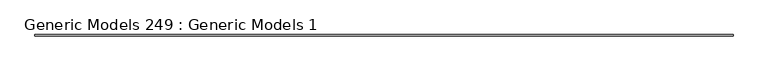
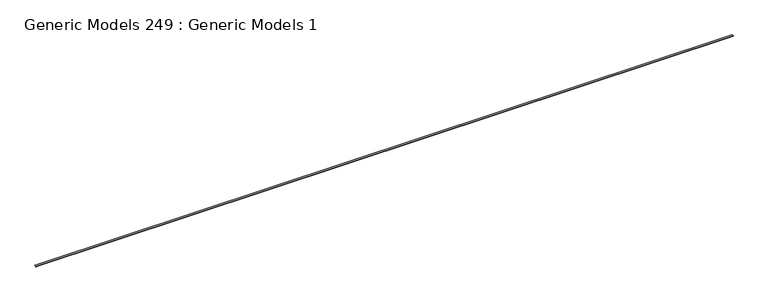
"""IFC4 building model written with IfcOpenShell, lengths in millimetres: proxy geometry, Generic Models 249 : Generic Models 1."""

import ifcopenshell
import ifcopenshell.guid

model = None  # the IFC model being written
_history = None  # IfcOwnerHistory: only IFC2X3 demands one
_inside = {}  # id of a spatial element -> (the spatial element, [elements in it])
_under = {}  # id of a project, library or spatial element -> (it, [spatial elements below it])
_declared = {}  # id of a project -> (the project, [libraries it declares])
_typed = {}  # id of a type object -> (the type object, [elements of that type])
_made_of = {}  # id of a material, layer set ... -> (it, [elements and type objects made of it])


def new_model(schema):
    """Start an empty IFC model of exactly this schema.

    Asked for "IFC4X3", IfcOpenShell would pick the latest addendum, in which some entities
    have other attributes; the version numbers below select the first issue.
    IFC2X3 requires an IfcOwnerHistory on every rooted entity: one is made here for all.
    """
    global model, _history
    if schema == "IFC4X3":
        model = ifcopenshell.file(schema_version=(4, 3, 0, 0))
    else:
        model = ifcopenshell.file(schema=schema)
    _inside.clear()
    _under.clear()
    _declared.clear()
    _typed.clear()
    _made_of.clear()
    _history = None
    if model.schema == "IFC2X3":
        org = make("IfcOrganization", Name="unknown")
        user = make(
            "IfcPersonAndOrganization",
            ThePerson=make("IfcPerson", FamilyName="unknown"),
            TheOrganization=org,
        )
        app = make(
            "IfcApplication",
            ApplicationDeveloper=org,
            Version="unknown",
            ApplicationFullName="unknown",
            ApplicationIdentifier="unknown",
        )
        _history = make(
            "IfcOwnerHistory",
            OwningUser=user,
            OwningApplication=app,
            ChangeAction="ADDED",
            CreationDate=0,
        )
    return model


def make(cls, **values):
    """One entity of the class cls with the attributes given. An attribute that is None is left unset."""
    return model.create_entity(
        cls, **{name: value for name, value in values.items() if value is not None}
    )


def rooted(cls, **values):
    """An entity with a GlobalId (a new one), such as an element, a storey or a relation."""
    return make(cls, GlobalId=ifcopenshell.guid.new(), OwnerHistory=_history, **values)


def si_unit(unit_type, name, prefix=None):
    """IfcSIUnit, for example si_unit("LENGTHUNIT", "METRE", prefix="MILLI")."""
    return make("IfcSIUnit", UnitType=unit_type, Prefix=prefix, Name=name)


def assignment(units):
    """IfcUnitAssignment: the units of a project."""
    return None if units is None else make("IfcUnitAssignment", Units=units)


def point(xyz):
    """IfcCartesianPoint."""
    return None if xyz is None else make("IfcCartesianPoint", Coordinates=xyz)


def direction(xyz):
    """IfcDirection."""
    return None if xyz is None else make("IfcDirection", DirectionRatios=xyz)


def frame(location, z_axis=None, x_axis=None):
    """IfcAxis2Placement3D, a coordinate frame: its origin and axes. An axis left out is left unset."""
    return make(
        "IfcAxis2Placement3D",
        Location=point(location),
        Axis=direction(z_axis),
        RefDirection=direction(x_axis),
    )


def origin():
    """The frame at (0, 0, 0) with its axes left unset."""
    return frame((0.0, 0.0, 0.0))


def place(relative_to, where):
    """IfcLocalPlacement: puts the frame where relative to a parent placement (None: the world)."""
    return make(
        "IfcLocalPlacement", PlacementRelTo=relative_to, RelativePlacement=where
    )


def context(
    kind, dimensions, precision=None, world=None, true_north=None, identifier=None
):
    """IfcGeometricRepresentationContext, for example the 3D "Model" context."""
    return make(
        "IfcGeometricRepresentationContext",
        ContextIdentifier=identifier,
        ContextType=kind,
        CoordinateSpaceDimension=dimensions,
        Precision=precision,
        WorldCoordinateSystem=world,
        TrueNorth=true_north,
    )


def project(units=None, contexts=None):
    """IfcProject with its units and contexts."""
    return rooted(
        "IfcProject",
        Name="project",
        RepresentationContexts=contexts,
        UnitsInContext=assignment(units),
    )


def spatial(cls, under=None, at=None, **own):
    """A site, building, storey or space (cls), placed at a placement, below another one or the project."""
    s = rooted(cls, ObjectPlacement=at, **own)
    if under is not None:
        _under.setdefault(under.id(), (under, []))[1].append(s)
    return s


def faces_of(points, faces, orient=None, outer=None):
    """IfcFace entities. A face is a list of loops; a loop is a list of indices into points, from 0.

    orient and outer hold one flag for each loop. By default every Orientation is true, the
    first loop of a face is its IfcFaceOuterBound and the others are IfcFaceBound.
    """
    made = []
    for i, loops in enumerate(faces):
        bounds = []
        for j, loop in enumerate(loops):
            is_outer = j == 0 if outer is None else outer[i][j]
            bounds.append(
                make(
                    "IfcFaceOuterBound" if is_outer else "IfcFaceBound",
                    Bound=make("IfcPolyLoop", Polygon=[points[k] for k in loop]),
                    Orientation=True if orient is None else orient[i][j],
                )
            )
        made.append(make("IfcFace", Bounds=bounds))
    return made


def faceted_brep(points, faces, orient=None, outer=None, voids=None):
    """IfcFacetedBrep: a solid bounded by flat faces; with voids (closed shells), ...WithVoids."""
    shared = [point(p) for p in points]
    hull = make("IfcClosedShell", CfsFaces=faces_of(shared, faces, orient, outer))
    if voids is None:
        return make("IfcFacetedBrep", Outer=hull)
    return make(
        "IfcFacetedBrepWithVoids",
        Outer=hull,
        Voids=[
            make(cls, CfsFaces=faces_of(shared, fs, o, b)) for cls, fs, o, b in voids
        ],
    )


def shape(context_of_items, identifier, shape_type, items):
    """IfcShapeRepresentation: the items that make up one representation, for example the "Body"."""
    return make(
        "IfcShapeRepresentation",
        ContextOfItems=context_of_items,
        RepresentationIdentifier=identifier,
        RepresentationType=shape_type,
        Items=items,
    )


def source(mapping_origin, context_of_items, identifier, shape_type, items):
    """IfcRepresentationMap: a shape defined once, which mapped items show again and again."""
    return make(
        "IfcRepresentationMap",
        MappingOrigin=mapping_origin,
        MappedRepresentation=shape(context_of_items, identifier, shape_type, items),
    )


def transform(
    local_origin,
    x_axis=None,
    y_axis=None,
    z_axis=None,
    scale=None,
    scale2=None,
    scale3=None,
    uniform=True,
):
    """IfcCartesianTransformationOperator3D, or its non-uniform kind. x_axis, y_axis, z_axis: its Axis1, 2, 3."""
    if uniform:
        return make(
            "IfcCartesianTransformationOperator3D",
            Axis1=direction(x_axis),
            Axis2=direction(y_axis),
            LocalOrigin=point(local_origin),
            Scale=scale,
            Axis3=direction(z_axis),
        )
    return make(
        "IfcCartesianTransformationOperator3DnonUniform",
        Axis1=direction(x_axis),
        Axis2=direction(y_axis),
        LocalOrigin=point(local_origin),
        Scale=scale,
        Axis3=direction(z_axis),
        Scale2=scale2,
        Scale3=scale3,
    )


def mapped(mapping_source, mapping_target):
    """IfcMappedItem: shows the shape of a source again, moved by a transform."""
    return make(
        "IfcMappedItem", MappingSource=mapping_source, MappingTarget=mapping_target
    )


def made_of(thing, what):
    """Note that an element or type object is made of a material, layer set ...; save() writes the relation."""
    if what is not None:
        _made_of.setdefault(what.id(), (what, []))[1].append(thing)
    return thing


def element(
    cls,
    number,
    at=None,
    inside=None,
    cuts=None,
    type_object=None,
    material=None,
    context=None,
    identifier="Body",
    shape_type=None,
    held_by="IfcProductDefinitionShape",
    body=None,
    shapes=None,
    **own,
):
    """One element of the class cls, such as IfcWall. Its Tag is "e" and its number.

    at: its placement. inside: the storey or other place that contains it. cuts: it is an
    opening in that element (IfcRelVoidsElement). A single representation is given by context,
    identifier, shape_type and body (its items); several are given by shapes. held_by: the class
    of the entity that holds the representations. save() writes the other relations.
    """
    e = rooted(cls, Tag="e%d" % number, ObjectPlacement=at, **own)
    if body is not None:
        shapes = [shape(context, identifier, shape_type, body)]
    if shapes is not None:
        e.Representation = make(held_by, Representations=shapes)
    if inside is not None:
        _inside.setdefault(inside.id(), (inside, []))[1].append(e)
    if cuts is not None:
        rooted(
            "IfcRelVoidsElement", RelatingBuildingElement=cuts, RelatedOpeningElement=e
        )
    if type_object is not None:
        _typed.setdefault(type_object.id(), (type_object, []))[1].append(e)
    return made_of(e, material)


def aggregate(whole, parts):
    """IfcRelAggregates: a whole, such as a stair, and the parts it consists of."""
    return rooted("IfcRelAggregates", RelatingObject=whole, RelatedObjects=parts)


def save(model, path):
    """Write the relations noted so far, then the file.

    IfcRelAggregates (storeys below a building ...), IfcRelContainedInSpatialStructure (elements
    in a storey), IfcRelDefinesByType, IfcRelAssociatesMaterial and IfcRelDeclares: one each for
    every whole, place, type object, material and project.
    """
    for whole, parts in _under.values():
        aggregate(whole, parts)
    for where, things in _inside.values():
        rooted(
            "IfcRelContainedInSpatialStructure",
            RelatedElements=things,
            RelatingStructure=where,
        )
    for kind, things in _typed.values():
        rooted("IfcRelDefinesByType", RelatedObjects=things, RelatingType=kind)
    for what, things in _made_of.values():
        rooted("IfcRelAssociatesMaterial", RelatedObjects=things, RelatingMaterial=what)
    for by, libraries in _declared.values():
        rooted("IfcRelDeclares", RelatingContext=by, RelatedDefinitions=libraries)
    model.write(path)


def generic_models_249_generic_models_1_f155bf51(model_context):
    return source(origin(), model_context, "Body", "Brep", [
        faceted_brep([(-5248.1628079, -20261.4171024, 126780.671), (-5248.1628079, -20261.4171024, 126802.896), (-5248.1628079, -20223.3171024, 126802.896), (-5248.1628079, -20223.3171024, 126801.626), (-5248.1628079, -20260.1471024, 126801.626), (-5248.1628079, -20260.1471024, 126781.941), (-5248.1628079, -20257.9373024, 126781.941), (-5248.1628079, -20257.9373024, 126783.6734564), (-5248.1628079, -20256.6673024, 126783.6734564), (-5248.1628079, -20256.6673024, 126780.671), (13801.8371921, -20261.4171024, 126780.671), (13801.8371921, -20256.6673024, 126780.671), (13801.8371921, -20256.6673024, 126783.6734564), (13801.8371921, -20257.9373024, 126783.6734564), (13801.8371921, -20257.9373024, 126781.941), (13801.8371921, -20260.1471024, 126781.941), (13801.8371921, -20260.1471024, 126801.626), (13801.8371921, -20223.3171024, 126801.626), (13801.8371921, -20223.3171024, 126802.896), (13801.8371921, -20261.4171024, 126802.896), (13593.8187142, -20223.3171024, 126802.896), (-5049.7812858, -20223.3171024, 126802.896), (13593.8187142, -20223.3171024, 126801.626), (-5049.7812858, -20223.3171024, 126801.626), (13593.8187142, -20260.1471024, 126801.626), (-5049.7812858, -20260.1471024, 126801.626), (13593.8187142, -20260.1471024, 126781.941), (-5049.7812858, -20260.1471024, 126781.941), (13593.8187142, -20257.9373024, 126781.941), (-5049.7812858, -20257.9373024, 126781.941), (-5049.7812858, -20257.9373024, 126783.6734564), (13593.8187142, -20257.9373024, 126783.6734564), (13593.8187142, -20256.6673024, 126783.6734564), (-5049.7812858, -20256.6673024, 126783.6734564), (13593.8187142, -20256.6673024, 126780.671), (-5049.7812858, -20256.6673024, 126780.671)], [[[0, 1, 2, 3, 4, 5, 6, 7, 8, 9]], [[10, 11, 12, 13, 14, 15, 16, 17, 18, 19]], [[1, 0, 10, 19]], [[2, 1, 19, 18, 20, 21]], [[3, 2, 21, 20, 18, 17, 22, 23]], [[4, 3, 23, 22, 17, 16, 24, 25]], [[5, 4, 25, 24, 16, 15, 26, 27]], [[6, 5, 27, 26, 15, 14, 28, 29]], [[8, 7, 30, 31, 13, 12, 32, 33]], [[9, 8, 33, 32, 12, 11, 34, 35]], [[0, 9, 35, 34, 11, 10]], [[7, 6, 29, 28, 14, 13, 31, 30]]]),
    ])


if __name__ == "__main__":
    model = new_model("IFC4")
    model_context = context("Model", 3, world=origin())
    ifc_project = project(units=[si_unit("LENGTHUNIT", "METRE", prefix="MILLI")], contexts=[model_context])
    site = spatial("IfcSite", under=ifc_project)
    building = spatial("IfcBuilding", under=site)
    placement = place(None, origin())
    generic_models_249_generic_models_1_shape = generic_models_249_generic_models_1_f155bf51(model_context)
    element("IfcBuildingElementProxy", 1, Name="Generic Models 249 : Generic Models 1", ObjectType="Generic Models 249 : Generic Models 1", at=placement, inside=building, context=model_context, shape_type="MappedRepresentation", body=[
        mapped(generic_models_249_generic_models_1_shape, transform((0.0, 0.0, 0.0), x_axis=(1.0, 0.0, 0.0), y_axis=(0.0, 1.0, 0.0), z_axis=(0.0, 0.0, 1.0))),
    ])
    save(model, "model.ifc")

# Revit data of these elements
# Element 1 (IfcBuildingElementProxy, "Generic Models 249 : Generic Models 1")
#   Materials on its faces: "_CONTINUOUS 16 GA. COPPER  J BEAD"
# Materials
#   "_CONTINUOUS 16 GA. COPPER  J BEAD": class "Generic", colour RGB 253 192 103, transparency 0, Cost = 0
